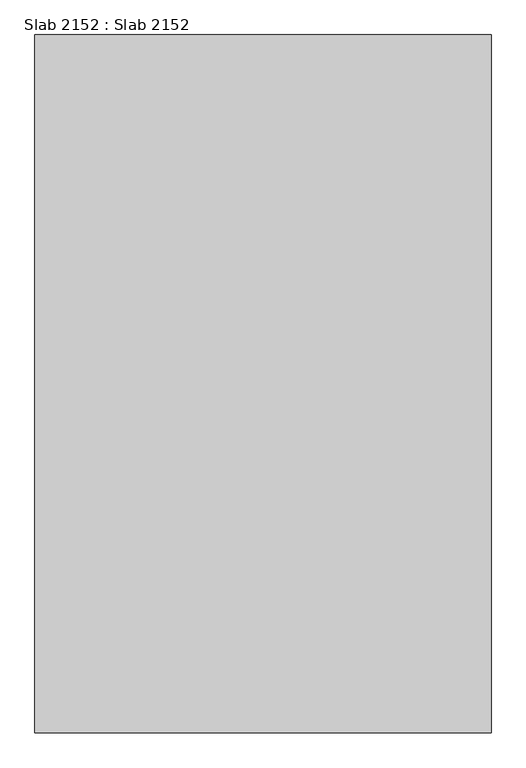
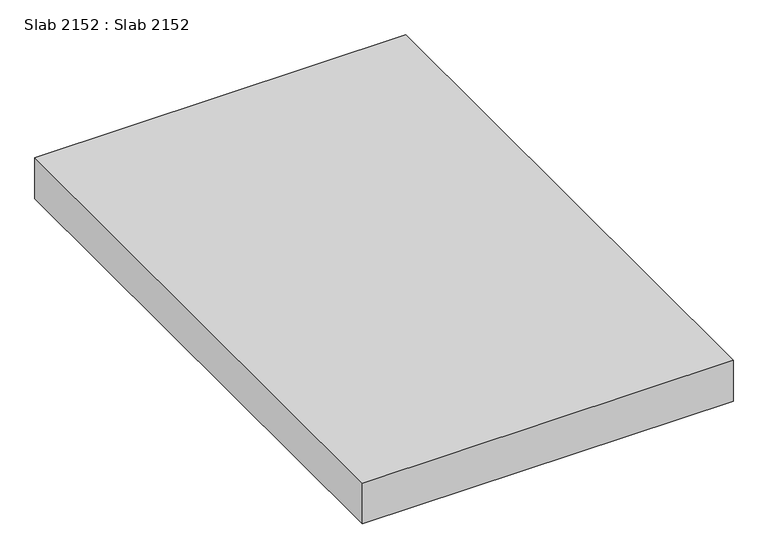
"""IFC4 building model written with IfcOpenShell, lengths in millimetres: proxy geometry, Slab 2152 : Slab 2152."""

from ifc_helpers import new_model, si_unit, frame, origin, place, context, project, spatial, polyline, outline, extrude, source, transform, mapped, element, save


def slab_2152_slab_2152_874da05e(model_context):
    return source(origin(), model_context, "Body", "SweptSolid", [
        extrude(outline(polyline([(-10261.8486328, 7982.1531721), (-11568.4300809, 7982.1531721), (-11568.4300809, 9982.1531721), (-10261.8486328, 9982.1531721), (-10261.8486328, 7982.1531721)])), frame((0.0, 0.0, 32467.2961275), z_axis=(0.0, 0.0, 1.0), x_axis=(1.0, 0.0, 0.0)), (0.0, 0.0, 1.0), 152.4078786),
    ])


if __name__ == "__main__":
    model = new_model("IFC4")
    model_context = context("Model", 3, world=origin())
    ifc_project = project(units=[si_unit("LENGTHUNIT", "METRE", prefix="MILLI")], contexts=[model_context])
    site = spatial("IfcSite", under=ifc_project)
    building = spatial("IfcBuilding", under=site)
    placement = place(None, origin())
    slab_2152_slab_2152_shape = slab_2152_slab_2152_874da05e(model_context)
    element("IfcBuildingElementProxy", 1, Name="Slab 2152 : Slab 2152", ObjectType="Slab 2152 : Slab 2152", at=placement, inside=building, context=model_context, shape_type="MappedRepresentation", body=[
        mapped(slab_2152_slab_2152_shape, transform((0.0, 0.0, 0.0), x_axis=(1.0, 0.0, 0.0), y_axis=(0.0, 1.0, 0.0), z_axis=(0.0, 0.0, 1.0))),
    ])
    save(model, "model.ifc")

# Revit data of these elements
# Type "Slab 2152 : Slab 2152"
#   NameOverride = "Slab"
# Element 1 (IfcBuildingElementProxy, "Slab 2152 : Slab 2152")
#   Materials on its faces: "4\" CONCRETE SLAB - SEE CIVIL DWGS"
# Materials
#   "4\" CONCRETE SLAB - SEE CIVIL DWGS": class "Unassigned", colour RGB 128 128 128, transparency 0, Cost = 0
